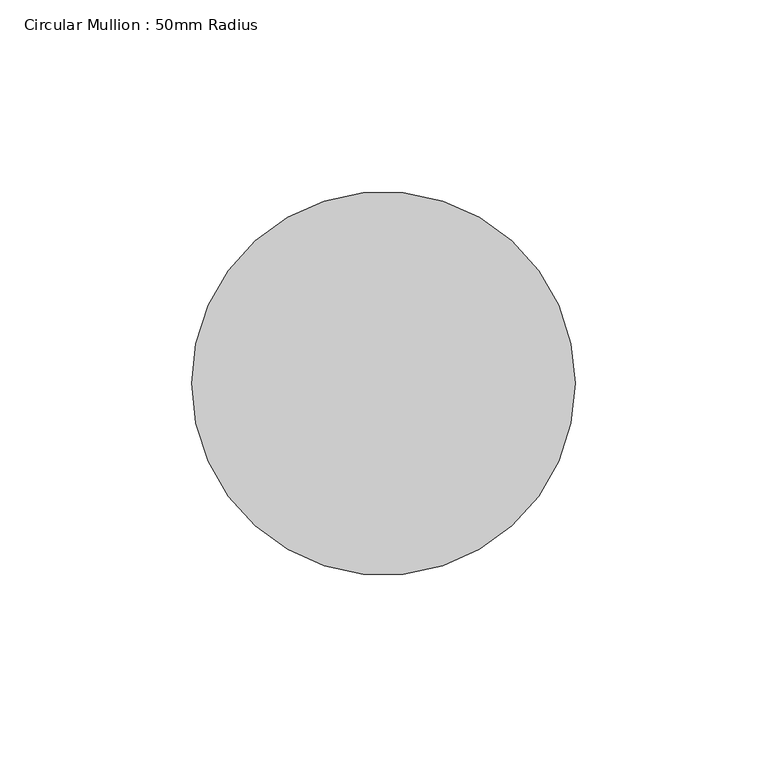
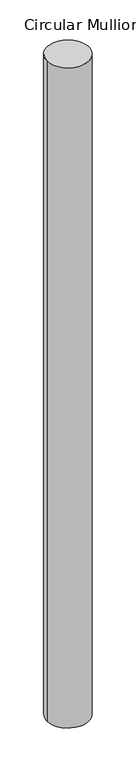
"""IFC4 building model written with IfcOpenShell, lengths in millimetres: member geometry, Circular Mullion : 50mm Radius."""

from ifc_helpers import new_model, si_unit, point, frame, origin, origin_2d, place, context, project, spatial, circle_curve, trimmed, segment, composite_curve, outline, extrude, source, transform, mapped, element, save


def circular_mullion_50mm_radius_2f5379a5(model_context):
    return source(origin(), model_context, "Body", "SweptSolid", [
        extrude(outline(composite_curve([segment(trimmed(circle_curve(origin_2d(), 50.0), [point((50.0, 0.0))], [point((-50.0, 0.0))], False, "CARTESIAN"), True, "CONTINUOUS"), segment(trimmed(circle_curve(origin_2d(), 50.0), [point((-50.0, 0.0))], [point((50.0, 0.0))], False, "CARTESIAN"), True, "CONTINUOUS")], self_intersect=False)), frame((0.0, 0.0, -1657.2217774), z_axis=(0.0, 0.0, 1.0), x_axis=(1.0, 0.0, 0.0)), (0.0, 0.0, 1.0), 1657.2217774),
    ])


if __name__ == "__main__":
    model = new_model("IFC4")
    model_context = context("Model", 3, world=origin())
    ifc_project = project(units=[si_unit("LENGTHUNIT", "METRE", prefix="MILLI")], contexts=[model_context])
    site = spatial("IfcSite", under=ifc_project)
    building = spatial("IfcBuilding", under=site)
    placement = place(None, origin())
    circular_mullion_50mm_radius_shape = circular_mullion_50mm_radius_2f5379a5(model_context)
    element("IfcMember", 1, ObjectType="Circular Mullion : 50mm Radius", at=placement, inside=building, context=model_context, shape_type="MappedRepresentation", body=[
        mapped(circular_mullion_50mm_radius_shape, transform((0.0, 0.0, 0.0), x_axis=(1.0, 0.0, 0.0), y_axis=(0.0, 1.0, 0.0), z_axis=(0.0, 0.0, 1.0))),
    ])
    save(model, "model.ifc")

# Revit data of these elements
# Type "Circular Mullion : 50mm Radius"
#   built-in parameter 1007350 = 0.164042 (stored number, unit not read)
# Element 1 (IfcMember, "Circular Mullion : 50mm Radius")
#   Materials on its faces: "Aluminium"
# Materials
#   "Aluminium": class "Metal", colour RGB 247 247 247, transparency 0, Description = "Aluminium 6061", Cost = 0
